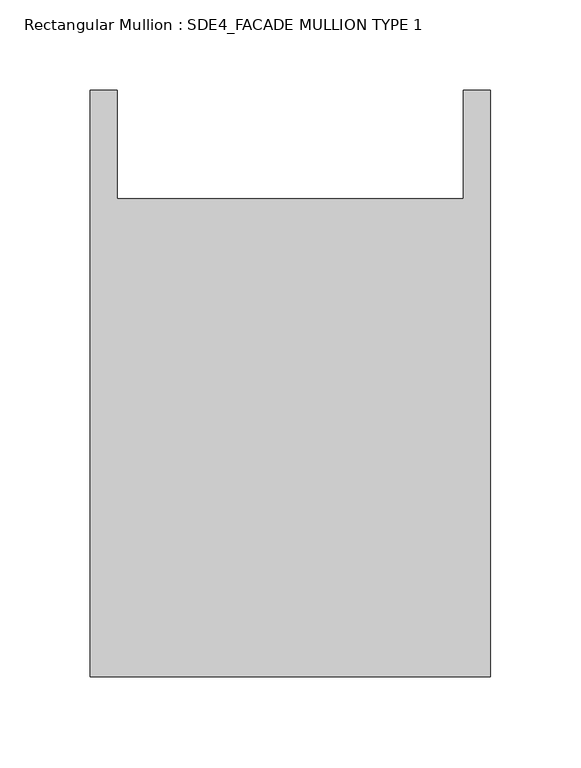
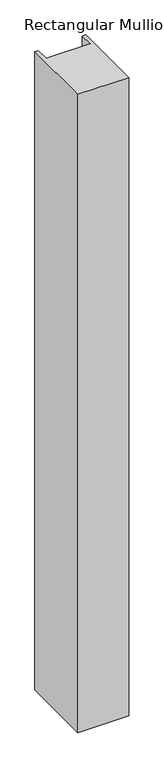
"""IFC4 building model written with IfcOpenShell, lengths in millimetres: member geometry, Rectangular Mullion : SDE4_FACADE MULLION TYPE 1."""

from ifc_helpers import new_model, si_unit, frame, origin, place, context, project, spatial, polyline, outline, extrude, source, transform, mapped, element, save


def rectangular_mullion_sde4_facade_mullion_type_1_b358935a(model_context):
    return source(origin(), model_context, "Body", "SweptSolid", [
        extrude(outline(polyline([(111.0, -132.5), (-111.0, -132.5), (-111.0, 192.5), (-96.0, 192.5), (-96.0, 132.5), (96.0, 132.5), (96.0, 192.5), (111.0, 192.5), (111.0, -132.5)])), frame((0.0, 0.0, -2950.0), z_axis=(0.0, 0.0, 1.0), x_axis=(1.0, 0.0, 0.0)), (0.0, 0.0, 1.0), 2950.0),
    ])


if __name__ == "__main__":
    model = new_model("IFC4")
    model_context = context("Model", 3, world=origin())
    ifc_project = project(units=[si_unit("LENGTHUNIT", "METRE", prefix="MILLI")], contexts=[model_context])
    site = spatial("IfcSite", under=ifc_project)
    building = spatial("IfcBuilding", under=site)
    placement = place(None, origin())
    rectangular_mullion_sde4_facade_mullion_type_1_shape = rectangular_mullion_sde4_facade_mullion_type_1_b358935a(model_context)
    element("IfcMember", 1, ObjectType="Rectangular Mullion : SDE4_FACADE MULLION TYPE 1", at=placement, inside=building, context=model_context, shape_type="MappedRepresentation", body=[
        mapped(rectangular_mullion_sde4_facade_mullion_type_1_shape, transform((0.0, 0.0, 0.0), x_axis=(1.0, 0.0, 0.0), y_axis=(0.0, 1.0, 0.0), z_axis=(0.0, 0.0, 1.0))),
    ])
    save(model, "model.ifc")

# Revit data of these elements
# Type "Rectangular Mullion : SDE4_FACADE MULLION TYPE 1"
#   built-in parameter 1007322 = 0.869423 (stored number, unit not read)
#   built-in parameter 1007321 = 0.364173 (stored number, unit not read)
#   built-in parameter 1007320 = 0.364173 (stored number, unit not read)
